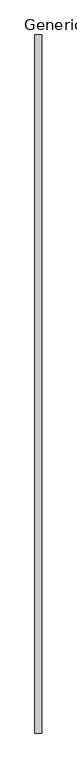
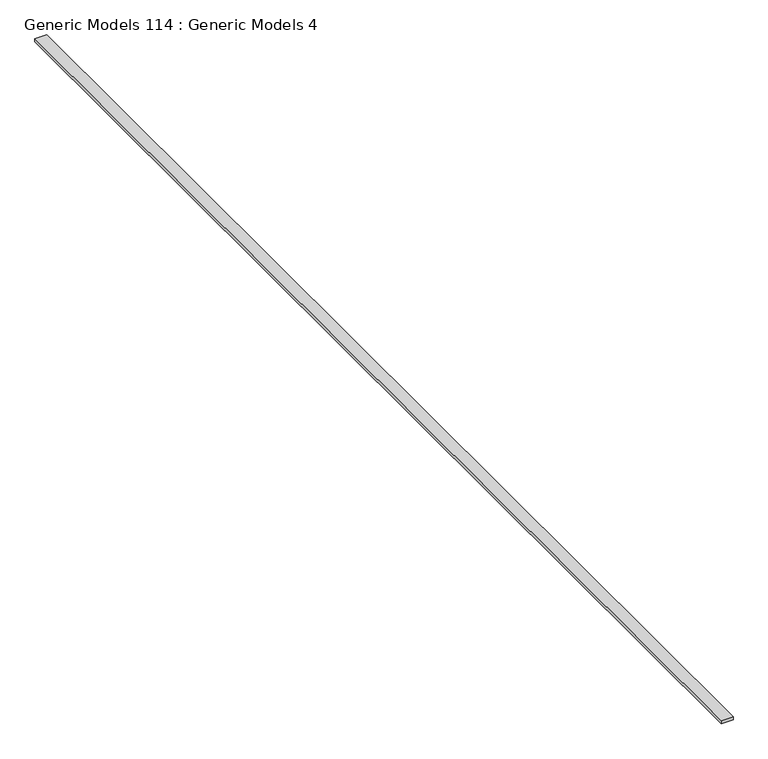
"""IFC4 building model written with IfcOpenShell, lengths in millimetres: proxy geometry, Generic Models 114 : Generic Models 4."""

from ifc_helpers import new_model, si_unit, frame, origin, place, context, project, spatial, polyline, outline, extrude, source, transform, mapped, element, save


def generic_models_114_generic_models_4_4d23e18a(model_context):
    return source(origin(), model_context, "Body", "SweptSolid", [
        extrude(outline(polyline([(-6470.8236296, -6864.9230338), (-6610.5236296, -6864.9230338), (-6610.5236296, 7054.2769662), (-6470.8236296, 7054.2769662), (-6470.8236296, -6864.9230338)])), frame((0.0, 0.0, 126211.4078034), z_axis=(0.0, 0.0, 1.0), x_axis=(1.0, 0.0, 0.0)), (0.0, 0.0, 1.0), 37.1331966),
    ])


if __name__ == "__main__":
    model = new_model("IFC4")
    model_context = context("Model", 3, world=origin())
    ifc_project = project(units=[si_unit("LENGTHUNIT", "METRE", prefix="MILLI")], contexts=[model_context])
    site = spatial("IfcSite", under=ifc_project)
    building = spatial("IfcBuilding", under=site)
    placement = place(None, origin())
    generic_models_114_generic_models_4_shape = generic_models_114_generic_models_4_4d23e18a(model_context)
    element("IfcBuildingElementProxy", 1, Name="Generic Models 114 : Generic Models 4", ObjectType="Generic Models 114 : Generic Models 4", at=placement, inside=building, context=model_context, shape_type="MappedRepresentation", body=[
        mapped(generic_models_114_generic_models_4_shape, transform((0.0, 0.0, 0.0), x_axis=(1.0, 0.0, 0.0), y_axis=(0.0, 1.0, 0.0), z_axis=(0.0, 0.0, 1.0))),
    ])
    save(model, "model.ifc")

# Revit data of these elements
# Element 1 (IfcBuildingElementProxy, "Generic Models 114 : Generic Models 4")
#   Materials on its faces: "_2X BLOCKING AS REQUIRED"
# Materials
#   "_2X BLOCKING AS REQUIRED": class "Generic", colour RGB 177 130 114, transparency 0, Cost = 0
